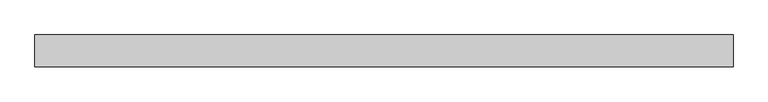
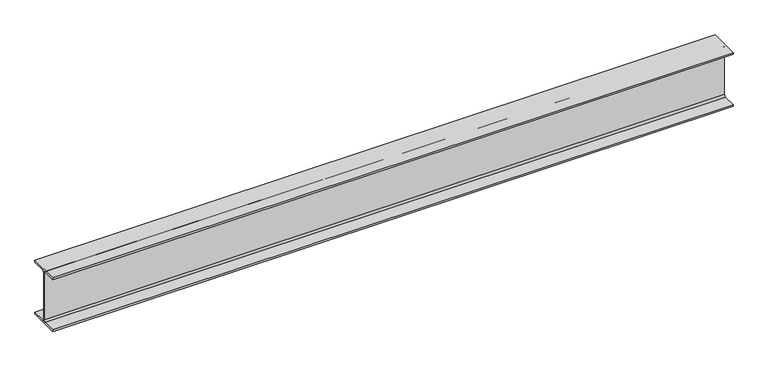
"""IFC4 building model written with IfcOpenShell, lengths in millimetres: beam geometry, Steel Beam_H-KSD3502 : H_SB_ASB_H-200x200x8x12."""

import ifcopenshell
import ifcopenshell.guid

model = None  # the IFC model being written
_history = None  # IfcOwnerHistory: only IFC2X3 demands one
_inside = {}  # id of a spatial element -> (the spatial element, [elements in it])
_under = {}  # id of a project, library or spatial element -> (it, [spatial elements below it])
_declared = {}  # id of a project -> (the project, [libraries it declares])
_typed = {}  # id of a type object -> (the type object, [elements of that type])
_made_of = {}  # id of a material, layer set ... -> (it, [elements and type objects made of it])


def new_model(schema):
    """Start an empty IFC model of exactly this schema.

    Asked for "IFC4X3", IfcOpenShell would pick the latest addendum, in which some entities
    have other attributes; the version numbers below select the first issue.
    IFC2X3 requires an IfcOwnerHistory on every rooted entity: one is made here for all.
    """
    global model, _history
    if schema == "IFC4X3":
        model = ifcopenshell.file(schema_version=(4, 3, 0, 0))
    else:
        model = ifcopenshell.file(schema=schema)
    _inside.clear()
    _under.clear()
    _declared.clear()
    _typed.clear()
    _made_of.clear()
    _history = None
    if model.schema == "IFC2X3":
        org = make("IfcOrganization", Name="unknown")
        user = make(
            "IfcPersonAndOrganization",
            ThePerson=make("IfcPerson", FamilyName="unknown"),
            TheOrganization=org,
        )
        app = make(
            "IfcApplication",
            ApplicationDeveloper=org,
            Version="unknown",
            ApplicationFullName="unknown",
            ApplicationIdentifier="unknown",
        )
        _history = make(
            "IfcOwnerHistory",
            OwningUser=user,
            OwningApplication=app,
            ChangeAction="ADDED",
            CreationDate=0,
        )
    return model


def make(cls, **values):
    """One entity of the class cls with the attributes given. An attribute that is None is left unset."""
    return model.create_entity(
        cls, **{name: value for name, value in values.items() if value is not None}
    )


def rooted(cls, **values):
    """An entity with a GlobalId (a new one), such as an element, a storey or a relation."""
    return make(cls, GlobalId=ifcopenshell.guid.new(), OwnerHistory=_history, **values)


def si_unit(unit_type, name, prefix=None):
    """IfcSIUnit, for example si_unit("LENGTHUNIT", "METRE", prefix="MILLI")."""
    return make("IfcSIUnit", UnitType=unit_type, Prefix=prefix, Name=name)


def assignment(units):
    """IfcUnitAssignment: the units of a project."""
    return None if units is None else make("IfcUnitAssignment", Units=units)


def point(xyz):
    """IfcCartesianPoint."""
    return None if xyz is None else make("IfcCartesianPoint", Coordinates=xyz)


def direction(xyz):
    """IfcDirection."""
    return None if xyz is None else make("IfcDirection", DirectionRatios=xyz)


def frame(location, z_axis=None, x_axis=None):
    """IfcAxis2Placement3D, a coordinate frame: its origin and axes. An axis left out is left unset."""
    return make(
        "IfcAxis2Placement3D",
        Location=point(location),
        Axis=direction(z_axis),
        RefDirection=direction(x_axis),
    )


def frame_2d(location, x_axis=None):
    """IfcAxis2Placement2D, a coordinate frame in the plane: its origin and x axis."""
    return make(
        "IfcAxis2Placement2D", Location=point(location), RefDirection=direction(x_axis)
    )


def origin():
    """The frame at (0, 0, 0) with its axes left unset."""
    return frame((0.0, 0.0, 0.0))


def place(relative_to, where):
    """IfcLocalPlacement: puts the frame where relative to a parent placement (None: the world)."""
    return make(
        "IfcLocalPlacement", PlacementRelTo=relative_to, RelativePlacement=where
    )


def context(
    kind, dimensions, precision=None, world=None, true_north=None, identifier=None
):
    """IfcGeometricRepresentationContext, for example the 3D "Model" context."""
    return make(
        "IfcGeometricRepresentationContext",
        ContextIdentifier=identifier,
        ContextType=kind,
        CoordinateSpaceDimension=dimensions,
        Precision=precision,
        WorldCoordinateSystem=world,
        TrueNorth=true_north,
    )


def project(units=None, contexts=None):
    """IfcProject with its units and contexts."""
    return rooted(
        "IfcProject",
        Name="project",
        RepresentationContexts=contexts,
        UnitsInContext=assignment(units),
    )


def spatial(cls, under=None, at=None, **own):
    """A site, building, storey or space (cls), placed at a placement, below another one or the project."""
    s = rooted(cls, ObjectPlacement=at, **own)
    if under is not None:
        _under.setdefault(under.id(), (under, []))[1].append(s)
    return s


def polyline(points):
    """IfcPolyline through the points."""
    return make("IfcPolyline", Points=[point(p) for p in points])


def circle_curve(where, radius):
    """IfcCircle in the frame where."""
    return make("IfcCircle", Position=where, Radius=radius)


def trimmed(basis, trim1, trim2, sense, master):
    """IfcTrimmedCurve: the piece of a basis curve between two trims."""
    return make(
        "IfcTrimmedCurve",
        BasisCurve=basis,
        Trim1=trim1,
        Trim2=trim2,
        SenseAgreement=sense,
        MasterRepresentation=master,
    )


def segment(curve, same_sense, transition):
    """IfcCompositeCurveSegment."""
    return make(
        "IfcCompositeCurveSegment",
        Transition=transition,
        SameSense=same_sense,
        ParentCurve=curve,
    )


def composite_curve(segments, self_intersect=None):
    """IfcCompositeCurve: segments joined end to end."""
    return make("IfcCompositeCurve", Segments=segments, SelfIntersect=self_intersect)


def outline(outer, holes=None, kind="AREA"):
    """IfcArbitraryClosedProfileDef: a profile drawn as a closed curve; with holes, ...WithVoids."""
    if holes is None:
        return make("IfcArbitraryClosedProfileDef", ProfileType=kind, OuterCurve=outer)
    return make(
        "IfcArbitraryProfileDefWithVoids",
        ProfileType=kind,
        OuterCurve=outer,
        InnerCurves=holes,
    )


def extrude(swept, where, along, depth):
    """IfcExtrudedAreaSolid: the profile swept, set in the frame where, extruded along a direction by depth."""
    return make(
        "IfcExtrudedAreaSolid",
        SweptArea=swept,
        Position=where,
        ExtrudedDirection=direction(along),
        Depth=depth,
    )


def shape(context_of_items, identifier, shape_type, items):
    """IfcShapeRepresentation: the items that make up one representation, for example the "Body"."""
    return make(
        "IfcShapeRepresentation",
        ContextOfItems=context_of_items,
        RepresentationIdentifier=identifier,
        RepresentationType=shape_type,
        Items=items,
    )


def source(mapping_origin, context_of_items, identifier, shape_type, items):
    """IfcRepresentationMap: a shape defined once, which mapped items show again and again."""
    return make(
        "IfcRepresentationMap",
        MappingOrigin=mapping_origin,
        MappedRepresentation=shape(context_of_items, identifier, shape_type, items),
    )


def transform(
    local_origin,
    x_axis=None,
    y_axis=None,
    z_axis=None,
    scale=None,
    scale2=None,
    scale3=None,
    uniform=True,
):
    """IfcCartesianTransformationOperator3D, or its non-uniform kind. x_axis, y_axis, z_axis: its Axis1, 2, 3."""
    if uniform:
        return make(
            "IfcCartesianTransformationOperator3D",
            Axis1=direction(x_axis),
            Axis2=direction(y_axis),
            LocalOrigin=point(local_origin),
            Scale=scale,
            Axis3=direction(z_axis),
        )
    return make(
        "IfcCartesianTransformationOperator3DnonUniform",
        Axis1=direction(x_axis),
        Axis2=direction(y_axis),
        LocalOrigin=point(local_origin),
        Scale=scale,
        Axis3=direction(z_axis),
        Scale2=scale2,
        Scale3=scale3,
    )


def mapped(mapping_source, mapping_target):
    """IfcMappedItem: shows the shape of a source again, moved by a transform."""
    return make(
        "IfcMappedItem", MappingSource=mapping_source, MappingTarget=mapping_target
    )


def made_of(thing, what):
    """Note that an element or type object is made of a material, layer set ...; save() writes the relation."""
    if what is not None:
        _made_of.setdefault(what.id(), (what, []))[1].append(thing)
    return thing


def element(
    cls,
    number,
    at=None,
    inside=None,
    cuts=None,
    type_object=None,
    material=None,
    context=None,
    identifier="Body",
    shape_type=None,
    held_by="IfcProductDefinitionShape",
    body=None,
    shapes=None,
    **own,
):
    """One element of the class cls, such as IfcWall. Its Tag is "e" and its number.

    at: its placement. inside: the storey or other place that contains it. cuts: it is an
    opening in that element (IfcRelVoidsElement). A single representation is given by context,
    identifier, shape_type and body (its items); several are given by shapes. held_by: the class
    of the entity that holds the representations. save() writes the other relations.
    """
    e = rooted(cls, Tag="e%d" % number, ObjectPlacement=at, **own)
    if body is not None:
        shapes = [shape(context, identifier, shape_type, body)]
    if shapes is not None:
        e.Representation = make(held_by, Representations=shapes)
    if inside is not None:
        _inside.setdefault(inside.id(), (inside, []))[1].append(e)
    if cuts is not None:
        rooted(
            "IfcRelVoidsElement", RelatingBuildingElement=cuts, RelatedOpeningElement=e
        )
    if type_object is not None:
        _typed.setdefault(type_object.id(), (type_object, []))[1].append(e)
    return made_of(e, material)


def aggregate(whole, parts):
    """IfcRelAggregates: a whole, such as a stair, and the parts it consists of."""
    return rooted("IfcRelAggregates", RelatingObject=whole, RelatedObjects=parts)


def save(model, path):
    """Write the relations noted so far, then the file.

    IfcRelAggregates (storeys below a building ...), IfcRelContainedInSpatialStructure (elements
    in a storey), IfcRelDefinesByType, IfcRelAssociatesMaterial and IfcRelDeclares: one each for
    every whole, place, type object, material and project.
    """
    for whole, parts in _under.values():
        aggregate(whole, parts)
    for where, things in _inside.values():
        rooted(
            "IfcRelContainedInSpatialStructure",
            RelatedElements=things,
            RelatingStructure=where,
        )
    for kind, things in _typed.values():
        rooted("IfcRelDefinesByType", RelatedObjects=things, RelatingType=kind)
    for what, things in _made_of.values():
        rooted("IfcRelAssociatesMaterial", RelatedObjects=things, RelatingMaterial=what)
    for by, libraries in _declared.values():
        rooted("IfcRelDeclares", RelatingContext=by, RelatedDefinitions=libraries)
    model.write(path)


def beam_c6904957(model_context):
    return source(origin(), model_context, "Body", "SweptSolid", [
        extrude(outline(composite_curve([segment(polyline([(82.5, -141.5), (82.5, -151.7), (-82.5, -151.7), (-82.5, -141.5), (-11.9, -141.5)]), True, "CONTINUOUS"), segment(trimmed(circle_curve(frame_2d((-11.9, -132.6)), 8.9), [point((-11.9, -141.5))], [point((-3.0, -132.6))], True, "CARTESIAN"), True, "CONTINUOUS"), segment(polyline([(-3.0, -132.6), (-3.0, 132.6)]), True, "CONTINUOUS"), segment(trimmed(circle_curve(frame_2d((-11.9, 132.6)), 8.9), [point((-3.0, 132.6))], [point((-11.9, 141.5))], True, "CARTESIAN"), True, "CONTINUOUS"), segment(polyline([(-11.9, 141.5), (-82.5, 141.5), (-82.5, 151.7), (82.5, 151.7), (82.5, 141.5), (11.9, 141.5)]), True, "CONTINUOUS"), segment(trimmed(circle_curve(frame_2d((11.9, 132.6)), 8.9), [point((11.9, 141.5))], [point((3.0, 132.6))], True, "CARTESIAN"), True, "CONTINUOUS"), segment(polyline([(3.0, 132.6), (3.0, -132.6)]), True, "CONTINUOUS"), segment(trimmed(circle_curve(frame_2d((11.9, -132.6)), 8.9), [point((3.0, -132.6))], [point((11.9, -141.5))], True, "CARTESIAN"), True, "CONTINUOUS"), segment(polyline([(11.9, -141.5), (82.5, -141.5)]), True, "CONTINUOUS")], self_intersect=False)), frame((-1780.1436483, 0.0, 0.0), z_axis=(1.0, 0.0, 0.0), x_axis=(0.0, 1.0, 0.0)), (0.0, 0.0, 1.0), 3630.9979746),
    ])


if __name__ == "__main__":
    model = new_model("IFC4")
    model_context = context("Model", 3, world=origin())
    ifc_project = project(units=[si_unit("LENGTHUNIT", "METRE", prefix="MILLI")], contexts=[model_context])
    site = spatial("IfcSite", under=ifc_project)
    building = spatial("IfcBuilding", under=site)
    placement = place(None, origin())
    beam_shape = beam_c6904957(model_context)
    element("IfcBeam", 1, ObjectType="Steel Beam_H-KSD3502 : H_SB_ASB_H-200x200x8x12", at=placement, inside=building, context=model_context, shape_type="MappedRepresentation", body=[
        mapped(beam_shape, transform((0.0, 0.0, 0.0), x_axis=(1.0, 0.0, 0.0), y_axis=(0.0, 1.0, 0.0), z_axis=(0.0, 0.0, 1.0))),
    ])
    save(model, "model.ifc")

# Revit data of these elements
# Type "Steel Beam_H-KSD3502 : H_SB_ASB_H-200x200x8x12"
#   Width = 20.0 cm
#   Web Thickness = 0.8 cm
#   Web Fillet = 1.3 cm
#   Warping Constant = 141376.0 cm⁶
#   Torsional Moment of Inertia = 26.2485 cm⁴
#   Torsional Modulus = 1.0 cm³
#   Section Area = 63.53 cm²
#   Plastic Modulus weak axis = 244.0 cm³
#   Plastic Modulus strong axis = 525.0 cm³
#   Perimeter = 1.16 m²/m
#   Nominal Weight = 49.90 kgf/m
#   Moment of Inertia weak axis = 1600.00 cm⁴
#   Moment of Inertia strong axis = 4720.00 cm⁴
#   Height = 20.0 cm
#   Flange Thickness = 1.2 cm
#   Elastic Modulus weak axis = 160.0 cm³
#   Elastic Modulus strong axis = 472.0 cm³
#   Centroid Vertical = 10.0 cm
#   Centroid Horizontal = 10.0 cm
#   Length [instance default] = 1.5240 m
#   Structural Material [instance default] = Steel, 45-345
#   Assembly Code = ""
# Element 1 (IfcBeam, "Steel Beam_H-KSD3502 : H_SB_ASB_H-200x200x8x12")
#   Structural Material = none
# Materials
#   "Steel, 45-345": class "Metal", colour RGB 189 187 185, transparency 0, Description = "Steel 345 MPa", Cost = 0
